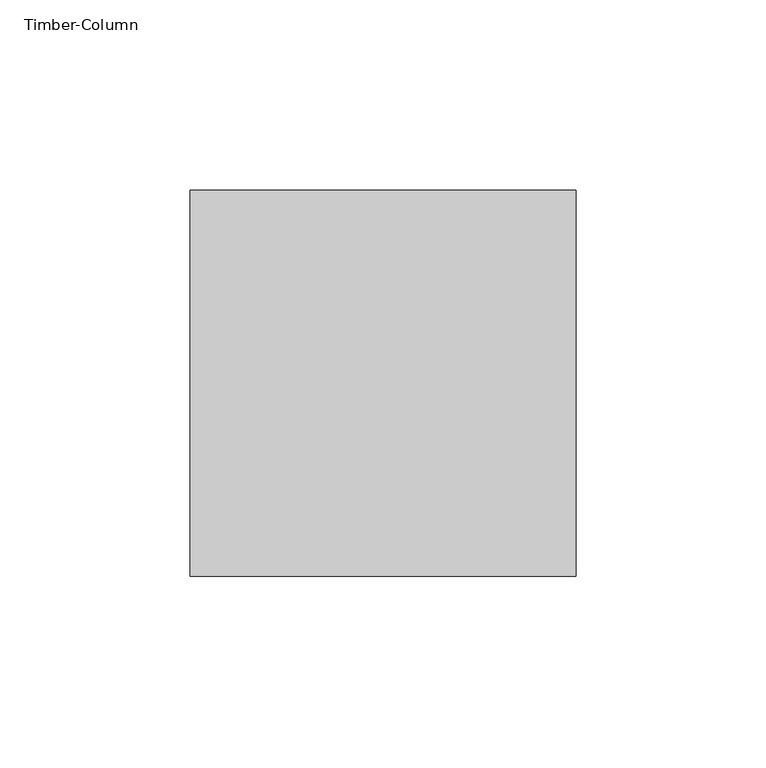
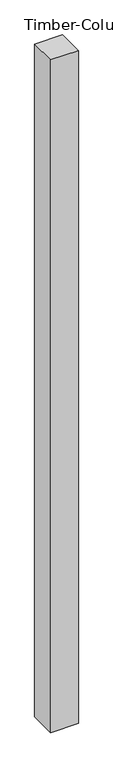
"""IFC4 building model written with IfcOpenShell, lengths in millimetres: column geometry, Timber-Column."""

from ifc_helpers import new_model, si_unit, frame, origin, place, context, project, spatial, polyline, outline, extrude, source, transform, mapped, element, save


def timber_column_b7e6a7b9(model_context):
    return source(origin(), model_context, "Body", "SweptSolid", [
        extrude(outline(polyline([(50.8, 50.8), (50.8, -50.8), (-50.8, -50.8), (-50.8, 50.8), (50.8, 50.8)])), frame((0.0, 0.0, 50.8), z_axis=(0.0, 0.0, 1.0), x_axis=(1.0, 0.0, 0.0)), (0.0, 0.0, 1.0), 2616.2),
    ])


if __name__ == "__main__":
    model = new_model("IFC4")
    model_context = context("Model", 3, world=origin())
    ifc_project = project(units=[si_unit("LENGTHUNIT", "METRE", prefix="MILLI")], contexts=[model_context])
    site = spatial("IfcSite", under=ifc_project)
    building = spatial("IfcBuilding", under=site)
    placement = place(None, origin())
    timber_column_shape = timber_column_b7e6a7b9(model_context)
    element("IfcColumn", 1, ObjectType="Timber-Column : BLDG 6241 Wall Struds 4\"x4\"", at=placement, inside=building, context=model_context, shape_type="MappedRepresentation", body=[
        mapped(timber_column_shape, transform((0.0, 0.0, 0.0), x_axis=(1.0, 0.0, 0.0), y_axis=(0.0, 1.0, 0.0), z_axis=(0.0, 0.0, 1.0))),
    ])
    save(model, "model.ifc")

# Revit data of these elements
# Type "Timber-Column : BLDG 6241 Wall Struds 4\"x4\""
#   Assembly Code = "B10"
#   A = 0.140625 SF
#   b = 0' - 4"
#   d = 0' - 4"
#   Structural Material [instance default] = Softwood, Lumber
# Element 1 (IfcColumn, "Timber-Column : BLDG 6241 Wall Struds 4\"x4\"")
#   Materials on its faces: "Softwood, Lumber"
# Materials
#   "Softwood, Lumber": class "Wood", colour RGB 223 192 134, transparency 0, Description = "Pinus Echinata", Cost = 0
